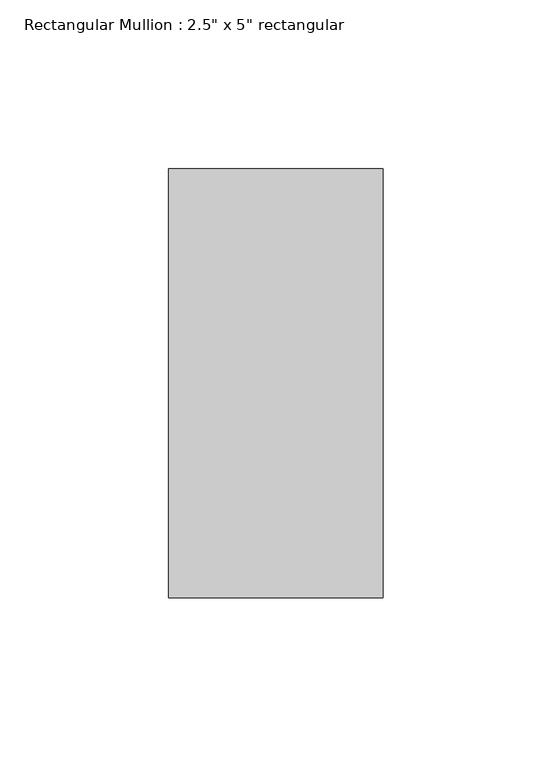
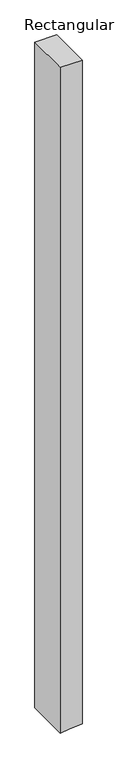
"""IFC4 building model written with IfcOpenShell, lengths in millimetres: member geometry."""

import ifcopenshell
import ifcopenshell.guid

model = None  # the IFC model being written
_history = None  # IfcOwnerHistory: only IFC2X3 demands one
_inside = {}  # id of a spatial element -> (the spatial element, [elements in it])
_under = {}  # id of a project, library or spatial element -> (it, [spatial elements below it])
_declared = {}  # id of a project -> (the project, [libraries it declares])
_typed = {}  # id of a type object -> (the type object, [elements of that type])
_made_of = {}  # id of a material, layer set ... -> (it, [elements and type objects made of it])


def new_model(schema):
    """Start an empty IFC model of exactly this schema.

    Asked for "IFC4X3", IfcOpenShell would pick the latest addendum, in which some entities
    have other attributes; the version numbers below select the first issue.
    IFC2X3 requires an IfcOwnerHistory on every rooted entity: one is made here for all.
    """
    global model, _history
    if schema == "IFC4X3":
        model = ifcopenshell.file(schema_version=(4, 3, 0, 0))
    else:
        model = ifcopenshell.file(schema=schema)
    _inside.clear()
    _under.clear()
    _declared.clear()
    _typed.clear()
    _made_of.clear()
    _history = None
    if model.schema == "IFC2X3":
        org = make("IfcOrganization", Name="unknown")
        user = make(
            "IfcPersonAndOrganization",
            ThePerson=make("IfcPerson", FamilyName="unknown"),
            TheOrganization=org,
        )
        app = make(
            "IfcApplication",
            ApplicationDeveloper=org,
            Version="unknown",
            ApplicationFullName="unknown",
            ApplicationIdentifier="unknown",
        )
        _history = make(
            "IfcOwnerHistory",
            OwningUser=user,
            OwningApplication=app,
            ChangeAction="ADDED",
            CreationDate=0,
        )
    return model


def make(cls, **values):
    """One entity of the class cls with the attributes given. An attribute that is None is left unset."""
    return model.create_entity(
        cls, **{name: value for name, value in values.items() if value is not None}
    )


def rooted(cls, **values):
    """An entity with a GlobalId (a new one), such as an element, a storey or a relation."""
    return make(cls, GlobalId=ifcopenshell.guid.new(), OwnerHistory=_history, **values)


def si_unit(unit_type, name, prefix=None):
    """IfcSIUnit, for example si_unit("LENGTHUNIT", "METRE", prefix="MILLI")."""
    return make("IfcSIUnit", UnitType=unit_type, Prefix=prefix, Name=name)


def assignment(units):
    """IfcUnitAssignment: the units of a project."""
    return None if units is None else make("IfcUnitAssignment", Units=units)


def point(xyz):
    """IfcCartesianPoint."""
    return None if xyz is None else make("IfcCartesianPoint", Coordinates=xyz)


def direction(xyz):
    """IfcDirection."""
    return None if xyz is None else make("IfcDirection", DirectionRatios=xyz)


def frame(location, z_axis=None, x_axis=None):
    """IfcAxis2Placement3D, a coordinate frame: its origin and axes. An axis left out is left unset."""
    return make(
        "IfcAxis2Placement3D",
        Location=point(location),
        Axis=direction(z_axis),
        RefDirection=direction(x_axis),
    )


def origin():
    """The frame at (0, 0, 0) with its axes left unset."""
    return frame((0.0, 0.0, 0.0))


def place(relative_to, where):
    """IfcLocalPlacement: puts the frame where relative to a parent placement (None: the world)."""
    return make(
        "IfcLocalPlacement", PlacementRelTo=relative_to, RelativePlacement=where
    )


def context(
    kind, dimensions, precision=None, world=None, true_north=None, identifier=None
):
    """IfcGeometricRepresentationContext, for example the 3D "Model" context."""
    return make(
        "IfcGeometricRepresentationContext",
        ContextIdentifier=identifier,
        ContextType=kind,
        CoordinateSpaceDimension=dimensions,
        Precision=precision,
        WorldCoordinateSystem=world,
        TrueNorth=true_north,
    )


def project(units=None, contexts=None):
    """IfcProject with its units and contexts."""
    return rooted(
        "IfcProject",
        Name="project",
        RepresentationContexts=contexts,
        UnitsInContext=assignment(units),
    )


def spatial(cls, under=None, at=None, **own):
    """A site, building, storey or space (cls), placed at a placement, below another one or the project."""
    s = rooted(cls, ObjectPlacement=at, **own)
    if under is not None:
        _under.setdefault(under.id(), (under, []))[1].append(s)
    return s


def polyline(points):
    """IfcPolyline through the points."""
    return make("IfcPolyline", Points=[point(p) for p in points])


def outline(outer, holes=None, kind="AREA"):
    """IfcArbitraryClosedProfileDef: a profile drawn as a closed curve; with holes, ...WithVoids."""
    if holes is None:
        return make("IfcArbitraryClosedProfileDef", ProfileType=kind, OuterCurve=outer)
    return make(
        "IfcArbitraryProfileDefWithVoids",
        ProfileType=kind,
        OuterCurve=outer,
        InnerCurves=holes,
    )


def extrude(swept, where, along, depth):
    """IfcExtrudedAreaSolid: the profile swept, set in the frame where, extruded along a direction by depth."""
    return make(
        "IfcExtrudedAreaSolid",
        SweptArea=swept,
        Position=where,
        ExtrudedDirection=direction(along),
        Depth=depth,
    )


def shape(context_of_items, identifier, shape_type, items):
    """IfcShapeRepresentation: the items that make up one representation, for example the "Body"."""
    return make(
        "IfcShapeRepresentation",
        ContextOfItems=context_of_items,
        RepresentationIdentifier=identifier,
        RepresentationType=shape_type,
        Items=items,
    )


def source(mapping_origin, context_of_items, identifier, shape_type, items):
    """IfcRepresentationMap: a shape defined once, which mapped items show again and again."""
    return make(
        "IfcRepresentationMap",
        MappingOrigin=mapping_origin,
        MappedRepresentation=shape(context_of_items, identifier, shape_type, items),
    )


def transform(
    local_origin,
    x_axis=None,
    y_axis=None,
    z_axis=None,
    scale=None,
    scale2=None,
    scale3=None,
    uniform=True,
):
    """IfcCartesianTransformationOperator3D, or its non-uniform kind. x_axis, y_axis, z_axis: its Axis1, 2, 3."""
    if uniform:
        return make(
            "IfcCartesianTransformationOperator3D",
            Axis1=direction(x_axis),
            Axis2=direction(y_axis),
            LocalOrigin=point(local_origin),
            Scale=scale,
            Axis3=direction(z_axis),
        )
    return make(
        "IfcCartesianTransformationOperator3DnonUniform",
        Axis1=direction(x_axis),
        Axis2=direction(y_axis),
        LocalOrigin=point(local_origin),
        Scale=scale,
        Axis3=direction(z_axis),
        Scale2=scale2,
        Scale3=scale3,
    )


def mapped(mapping_source, mapping_target):
    """IfcMappedItem: shows the shape of a source again, moved by a transform."""
    return make(
        "IfcMappedItem", MappingSource=mapping_source, MappingTarget=mapping_target
    )


def made_of(thing, what):
    """Note that an element or type object is made of a material, layer set ...; save() writes the relation."""
    if what is not None:
        _made_of.setdefault(what.id(), (what, []))[1].append(thing)
    return thing


def element(
    cls,
    number,
    at=None,
    inside=None,
    cuts=None,
    type_object=None,
    material=None,
    context=None,
    identifier="Body",
    shape_type=None,
    held_by="IfcProductDefinitionShape",
    body=None,
    shapes=None,
    **own,
):
    """One element of the class cls, such as IfcWall. Its Tag is "e" and its number.

    at: its placement. inside: the storey or other place that contains it. cuts: it is an
    opening in that element (IfcRelVoidsElement). A single representation is given by context,
    identifier, shape_type and body (its items); several are given by shapes. held_by: the class
    of the entity that holds the representations. save() writes the other relations.
    """
    e = rooted(cls, Tag="e%d" % number, ObjectPlacement=at, **own)
    if body is not None:
        shapes = [shape(context, identifier, shape_type, body)]
    if shapes is not None:
        e.Representation = make(held_by, Representations=shapes)
    if inside is not None:
        _inside.setdefault(inside.id(), (inside, []))[1].append(e)
    if cuts is not None:
        rooted(
            "IfcRelVoidsElement", RelatingBuildingElement=cuts, RelatedOpeningElement=e
        )
    if type_object is not None:
        _typed.setdefault(type_object.id(), (type_object, []))[1].append(e)
    return made_of(e, material)


def aggregate(whole, parts):
    """IfcRelAggregates: a whole, such as a stair, and the parts it consists of."""
    return rooted("IfcRelAggregates", RelatingObject=whole, RelatedObjects=parts)


def save(model, path):
    """Write the relations noted so far, then the file.

    IfcRelAggregates (storeys below a building ...), IfcRelContainedInSpatialStructure (elements
    in a storey), IfcRelDefinesByType, IfcRelAssociatesMaterial and IfcRelDeclares: one each for
    every whole, place, type object, material and project.
    """
    for whole, parts in _under.values():
        aggregate(whole, parts)
    for where, things in _inside.values():
        rooted(
            "IfcRelContainedInSpatialStructure",
            RelatedElements=things,
            RelatingStructure=where,
        )
    for kind, things in _typed.values():
        rooted("IfcRelDefinesByType", RelatedObjects=things, RelatingType=kind)
    for what, things in _made_of.values():
        rooted("IfcRelAssociatesMaterial", RelatedObjects=things, RelatingMaterial=what)
    for by, libraries in _declared.values():
        rooted("IfcRelDeclares", RelatingContext=by, RelatedDefinitions=libraries)
    model.write(path)


def member_dbe99c52(model_context):
    return source(origin(), model_context, "Body", "SweptSolid", [
        extrude(outline(polyline([(0.0, 31.75), (0.0, -31.75), (-2042.2724047, -31.75), (-2039.5298379, -6.9912306), (-2035.2384125, 31.75), (0.0, 31.75)])), frame((0.0, -63.5, 0.0), z_axis=(0.0, 1.0, 0.0), x_axis=(0.0, 0.0, 1.0)), (0.0, 0.0, 1.0), 127.0),
    ])


if __name__ == "__main__":
    model = new_model("IFC4")
    model_context = context("Model", 3, world=origin())
    ifc_project = project(units=[si_unit("LENGTHUNIT", "METRE", prefix="MILLI")], contexts=[model_context])
    site = spatial("IfcSite", under=ifc_project)
    building = spatial("IfcBuilding", under=site)
    placement = place(None, origin())
    member_shape = member_dbe99c52(model_context)
    element("IfcMember", 1, ObjectType="Rectangular Mullion : 2.5\" x 5\" rectangular", at=placement, inside=building, context=model_context, shape_type="MappedRepresentation", body=[
        mapped(member_shape, transform((0.0, 0.0, 0.0), x_axis=(1.0, 0.0, 0.0), y_axis=(0.0, 1.0, 0.0), z_axis=(0.0, 0.0, 1.0))),
    ])
    save(model, "model.ifc")

# Revit data of these elements
# Type "Rectangular Mullion : 2.5\" x 5\" rectangular"
#   built-in parameter 1007304 = 0.416667 (stored number, unit not read)
#   built-in parameter 1007301 = 0.104167 (stored number, unit not read)
#   built-in parameter 1007300 = 0.104167 (stored number, unit not read)
# Element 1 (IfcMember, "Rectangular Mullion : 2.5\" x 5\" rectangular")
#   Materials on its faces: "Aluminum"
# Materials
#   "Aluminum": class "Metal", colour RGB 247 247 247, transparency 0, Description = "Aluminum 6061", Cost = 0
